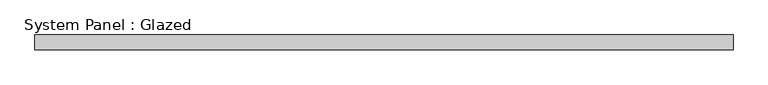
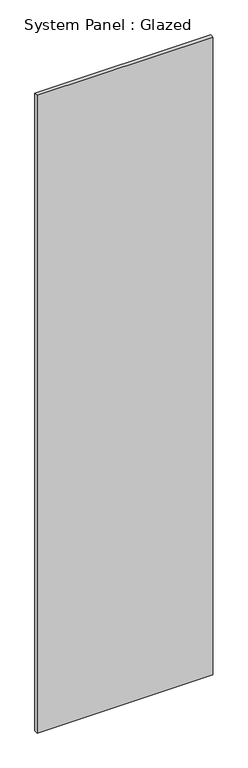
"""IFC4 building model written with IfcOpenShell, lengths in millimetres: plate geometry, System Panel : Glazed."""

import ifcopenshell
import ifcopenshell.guid

model = None  # the IFC model being written
_history = None  # IfcOwnerHistory: only IFC2X3 demands one
_inside = {}  # id of a spatial element -> (the spatial element, [elements in it])
_under = {}  # id of a project, library or spatial element -> (it, [spatial elements below it])
_declared = {}  # id of a project -> (the project, [libraries it declares])
_typed = {}  # id of a type object -> (the type object, [elements of that type])
_made_of = {}  # id of a material, layer set ... -> (it, [elements and type objects made of it])


def new_model(schema):
    """Start an empty IFC model of exactly this schema.

    Asked for "IFC4X3", IfcOpenShell would pick the latest addendum, in which some entities
    have other attributes; the version numbers below select the first issue.
    IFC2X3 requires an IfcOwnerHistory on every rooted entity: one is made here for all.
    """
    global model, _history
    if schema == "IFC4X3":
        model = ifcopenshell.file(schema_version=(4, 3, 0, 0))
    else:
        model = ifcopenshell.file(schema=schema)
    _inside.clear()
    _under.clear()
    _declared.clear()
    _typed.clear()
    _made_of.clear()
    _history = None
    if model.schema == "IFC2X3":
        org = make("IfcOrganization", Name="unknown")
        user = make(
            "IfcPersonAndOrganization",
            ThePerson=make("IfcPerson", FamilyName="unknown"),
            TheOrganization=org,
        )
        app = make(
            "IfcApplication",
            ApplicationDeveloper=org,
            Version="unknown",
            ApplicationFullName="unknown",
            ApplicationIdentifier="unknown",
        )
        _history = make(
            "IfcOwnerHistory",
            OwningUser=user,
            OwningApplication=app,
            ChangeAction="ADDED",
            CreationDate=0,
        )
    return model


def make(cls, **values):
    """One entity of the class cls with the attributes given. An attribute that is None is left unset."""
    return model.create_entity(
        cls, **{name: value for name, value in values.items() if value is not None}
    )


def rooted(cls, **values):
    """An entity with a GlobalId (a new one), such as an element, a storey or a relation."""
    return make(cls, GlobalId=ifcopenshell.guid.new(), OwnerHistory=_history, **values)


def si_unit(unit_type, name, prefix=None):
    """IfcSIUnit, for example si_unit("LENGTHUNIT", "METRE", prefix="MILLI")."""
    return make("IfcSIUnit", UnitType=unit_type, Prefix=prefix, Name=name)


def assignment(units):
    """IfcUnitAssignment: the units of a project."""
    return None if units is None else make("IfcUnitAssignment", Units=units)


def point(xyz):
    """IfcCartesianPoint."""
    return None if xyz is None else make("IfcCartesianPoint", Coordinates=xyz)


def direction(xyz):
    """IfcDirection."""
    return None if xyz is None else make("IfcDirection", DirectionRatios=xyz)


def frame(location, z_axis=None, x_axis=None):
    """IfcAxis2Placement3D, a coordinate frame: its origin and axes. An axis left out is left unset."""
    return make(
        "IfcAxis2Placement3D",
        Location=point(location),
        Axis=direction(z_axis),
        RefDirection=direction(x_axis),
    )


def origin():
    """The frame at (0, 0, 0) with its axes left unset."""
    return frame((0.0, 0.0, 0.0))


def origin_with_axes():
    """The frame at (0, 0, 0) with the z axis (0, 0, 1) and the x axis (1, 0, 0) written out."""
    return frame((0.0, 0.0, 0.0), z_axis=(0.0, 0.0, 1.0), x_axis=(1.0, 0.0, 0.0))


def place(relative_to, where):
    """IfcLocalPlacement: puts the frame where relative to a parent placement (None: the world)."""
    return make(
        "IfcLocalPlacement", PlacementRelTo=relative_to, RelativePlacement=where
    )


def context(
    kind, dimensions, precision=None, world=None, true_north=None, identifier=None
):
    """IfcGeometricRepresentationContext, for example the 3D "Model" context."""
    return make(
        "IfcGeometricRepresentationContext",
        ContextIdentifier=identifier,
        ContextType=kind,
        CoordinateSpaceDimension=dimensions,
        Precision=precision,
        WorldCoordinateSystem=world,
        TrueNorth=true_north,
    )


def project(units=None, contexts=None):
    """IfcProject with its units and contexts."""
    return rooted(
        "IfcProject",
        Name="project",
        RepresentationContexts=contexts,
        UnitsInContext=assignment(units),
    )


def spatial(cls, under=None, at=None, **own):
    """A site, building, storey or space (cls), placed at a placement, below another one or the project."""
    s = rooted(cls, ObjectPlacement=at, **own)
    if under is not None:
        _under.setdefault(under.id(), (under, []))[1].append(s)
    return s


def polyline(points):
    """IfcPolyline through the points."""
    return make("IfcPolyline", Points=[point(p) for p in points])


def outline(outer, holes=None, kind="AREA"):
    """IfcArbitraryClosedProfileDef: a profile drawn as a closed curve; with holes, ...WithVoids."""
    if holes is None:
        return make("IfcArbitraryClosedProfileDef", ProfileType=kind, OuterCurve=outer)
    return make(
        "IfcArbitraryProfileDefWithVoids",
        ProfileType=kind,
        OuterCurve=outer,
        InnerCurves=holes,
    )


def extrude(swept, where, along, depth):
    """IfcExtrudedAreaSolid: the profile swept, set in the frame where, extruded along a direction by depth."""
    return make(
        "IfcExtrudedAreaSolid",
        SweptArea=swept,
        Position=where,
        ExtrudedDirection=direction(along),
        Depth=depth,
    )


def shape(context_of_items, identifier, shape_type, items):
    """IfcShapeRepresentation: the items that make up one representation, for example the "Body"."""
    return make(
        "IfcShapeRepresentation",
        ContextOfItems=context_of_items,
        RepresentationIdentifier=identifier,
        RepresentationType=shape_type,
        Items=items,
    )


def source(mapping_origin, context_of_items, identifier, shape_type, items):
    """IfcRepresentationMap: a shape defined once, which mapped items show again and again."""
    return make(
        "IfcRepresentationMap",
        MappingOrigin=mapping_origin,
        MappedRepresentation=shape(context_of_items, identifier, shape_type, items),
    )


def transform(
    local_origin,
    x_axis=None,
    y_axis=None,
    z_axis=None,
    scale=None,
    scale2=None,
    scale3=None,
    uniform=True,
):
    """IfcCartesianTransformationOperator3D, or its non-uniform kind. x_axis, y_axis, z_axis: its Axis1, 2, 3."""
    if uniform:
        return make(
            "IfcCartesianTransformationOperator3D",
            Axis1=direction(x_axis),
            Axis2=direction(y_axis),
            LocalOrigin=point(local_origin),
            Scale=scale,
            Axis3=direction(z_axis),
        )
    return make(
        "IfcCartesianTransformationOperator3DnonUniform",
        Axis1=direction(x_axis),
        Axis2=direction(y_axis),
        LocalOrigin=point(local_origin),
        Scale=scale,
        Axis3=direction(z_axis),
        Scale2=scale2,
        Scale3=scale3,
    )


def mapped(mapping_source, mapping_target):
    """IfcMappedItem: shows the shape of a source again, moved by a transform."""
    return make(
        "IfcMappedItem", MappingSource=mapping_source, MappingTarget=mapping_target
    )


def made_of(thing, what):
    """Note that an element or type object is made of a material, layer set ...; save() writes the relation."""
    if what is not None:
        _made_of.setdefault(what.id(), (what, []))[1].append(thing)
    return thing


def element(
    cls,
    number,
    at=None,
    inside=None,
    cuts=None,
    type_object=None,
    material=None,
    context=None,
    identifier="Body",
    shape_type=None,
    held_by="IfcProductDefinitionShape",
    body=None,
    shapes=None,
    **own,
):
    """One element of the class cls, such as IfcWall. Its Tag is "e" and its number.

    at: its placement. inside: the storey or other place that contains it. cuts: it is an
    opening in that element (IfcRelVoidsElement). A single representation is given by context,
    identifier, shape_type and body (its items); several are given by shapes. held_by: the class
    of the entity that holds the representations. save() writes the other relations.
    """
    e = rooted(cls, Tag="e%d" % number, ObjectPlacement=at, **own)
    if body is not None:
        shapes = [shape(context, identifier, shape_type, body)]
    if shapes is not None:
        e.Representation = make(held_by, Representations=shapes)
    if inside is not None:
        _inside.setdefault(inside.id(), (inside, []))[1].append(e)
    if cuts is not None:
        rooted(
            "IfcRelVoidsElement", RelatingBuildingElement=cuts, RelatedOpeningElement=e
        )
    if type_object is not None:
        _typed.setdefault(type_object.id(), (type_object, []))[1].append(e)
    return made_of(e, material)


def aggregate(whole, parts):
    """IfcRelAggregates: a whole, such as a stair, and the parts it consists of."""
    return rooted("IfcRelAggregates", RelatingObject=whole, RelatedObjects=parts)


def save(model, path):
    """Write the relations noted so far, then the file.

    IfcRelAggregates (storeys below a building ...), IfcRelContainedInSpatialStructure (elements
    in a storey), IfcRelDefinesByType, IfcRelAssociatesMaterial and IfcRelDeclares: one each for
    every whole, place, type object, material and project.
    """
    for whole, parts in _under.values():
        aggregate(whole, parts)
    for where, things in _inside.values():
        rooted(
            "IfcRelContainedInSpatialStructure",
            RelatedElements=things,
            RelatingStructure=where,
        )
    for kind, things in _typed.values():
        rooted("IfcRelDefinesByType", RelatedObjects=things, RelatingType=kind)
    for what, things in _made_of.values():
        rooted("IfcRelAssociatesMaterial", RelatedObjects=things, RelatingMaterial=what)
    for by, libraries in _declared.values():
        rooted("IfcRelDeclares", RelatingContext=by, RelatedDefinitions=libraries)
    model.write(path)


def system_panel_glazed_26f8e022(model_context):
    return source(origin(), model_context, "Body", "SweptSolid", [
        extrude(outline(polyline([(603.7494819, 19.05), (-603.7494819, 19.05), (-603.7494819, 44.45), (603.7494819, 44.45), (603.7494819, 19.05)])), origin_with_axes(), (0.0, 0.0, 1.0), 4629.15),
    ])


if __name__ == "__main__":
    model = new_model("IFC4")
    model_context = context("Model", 3, world=origin())
    ifc_project = project(units=[si_unit("LENGTHUNIT", "METRE", prefix="MILLI")], contexts=[model_context])
    site = spatial("IfcSite", under=ifc_project)
    building = spatial("IfcBuilding", under=site)
    placement = place(None, origin())
    system_panel_glazed_shape = system_panel_glazed_26f8e022(model_context)
    element("IfcPlate", 1, ObjectType="System Panel : Glazed", at=placement, inside=building, context=model_context, shape_type="MappedRepresentation", body=[
        mapped(system_panel_glazed_shape, transform((0.0, 0.0, 0.0), x_axis=(1.0, 0.0, 0.0), y_axis=(0.0, 1.0, 0.0), z_axis=(0.0, 0.0, 1.0))),
    ])
    save(model, "model.ifc")

# Revit data of these elements
# Type "System Panel : Glazed"
#   Construction Type Id = "GSP4R"
#   Analytic Construction = "1/8 in Pilkington single glazing"
#   Visual Light Transmittance = 0.9
#   Solar Heat Gain Coefficient = 0.86
#   Heat Transfer Coefficient (U) = 1.18115 BTU/(h·ft²·°F)
#   Define Thermal Properties by = 1
# Element 1 (IfcPlate, "System Panel : Glazed")
#   Materials on its faces: "Glass"
# Materials
#   "Glass": class "Glass", colour RGB 0 128 192, transparency 0.75, Description = "Soda Lime Glass", Cost = 0
